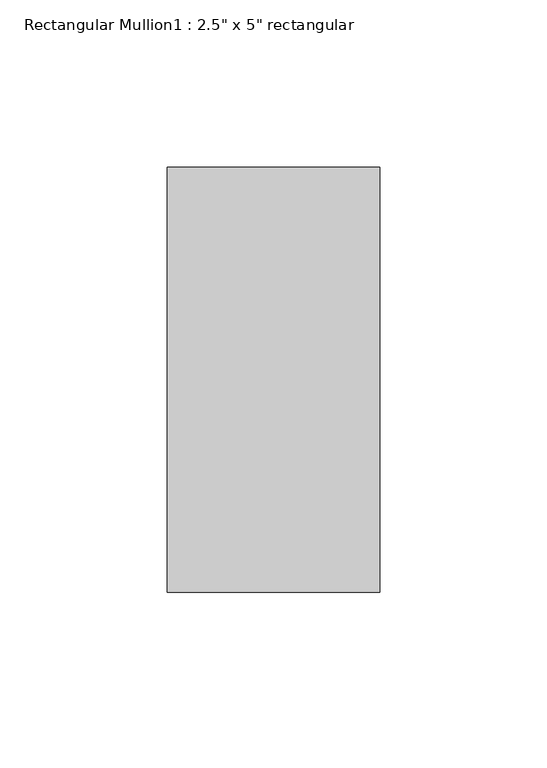
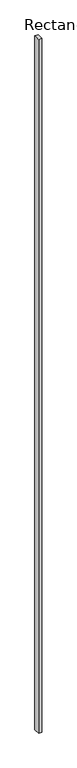
"""IFC4 building model written with IfcOpenShell, lengths in millimetres: member geometry."""

from ifc_helpers import new_model, si_unit, frame, origin, place, context, project, spatial, polyline, outline, extrude, source, transform, mapped, element, save


def member_bd9c79d2(model_context):
    return source(origin(), model_context, "Body", "SweptSolid", [
        extrude(outline(polyline([(0.0, 63.5), (0.0, -63.5), (-63.5, -63.5), (-63.5, 63.5), (0.0, 63.5)])), frame((0.0, 0.0, -14960.6), z_axis=(0.0, 0.0, 1.0), x_axis=(1.0, 0.0, 0.0)), (0.0, 0.0, 1.0), 14960.6),
    ])


if __name__ == "__main__":
    model = new_model("IFC4")
    model_context = context("Model", 3, world=origin())
    ifc_project = project(units=[si_unit("LENGTHUNIT", "METRE", prefix="MILLI")], contexts=[model_context])
    site = spatial("IfcSite", under=ifc_project)
    building = spatial("IfcBuilding", under=site)
    placement = place(None, origin())
    member_shape = member_bd9c79d2(model_context)
    element("IfcMember", 1, ObjectType="Rectangular Mullion1 : 2.5\" x 5\" rectangular", at=placement, inside=building, context=model_context, shape_type="MappedRepresentation", body=[
        mapped(member_shape, transform((0.0, 0.0, 0.0), x_axis=(1.0, 0.0, 0.0), y_axis=(0.0, 1.0, 0.0), z_axis=(0.0, 0.0, 1.0))),
    ])
    save(model, "model.ifc")

# Revit data of these elements
# Type "Rectangular Mullion1 : 2.5\" x 5\" rectangular"
#   built-in parameter 1007304 = 0.416667 (stored number, unit not read)
#   built-in parameter 1007301 = 0.104167 (stored number, unit not read)
#   built-in parameter 1007300 = 0.104167 (stored number, unit not read)
# Element 1 (IfcMember, "Rectangular Mullion1 : 2.5\" x 5\" rectangular")
#   Materials on its faces: "support-frame"
# Materials
#   "support-frame": class "Unassigned", colour RGB 233 233 233, transparency 0, Cost = 0
